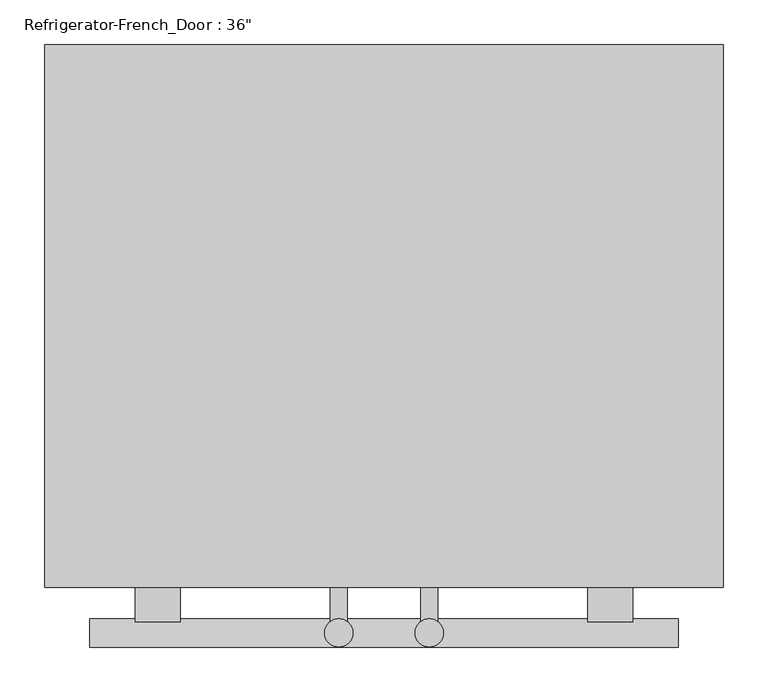
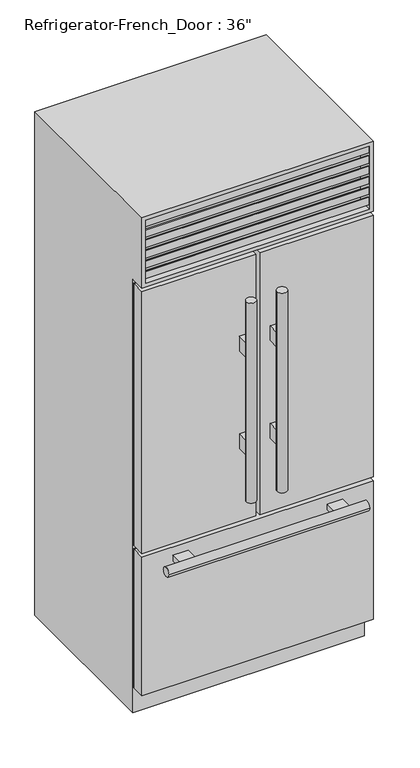
"""IFC4 building model written with IfcOpenShell, lengths in millimetres: proxy geometry."""

from ifc_helpers import new_model, si_unit, frame, origin, place, context, project, spatial, polyline, circle_curve, ellipse_curve, outline, extrude, faceted_brep, source, transform, mapped, element, save
from ifc_brep_helpers import plane_surface, cylinder_surface, advanced_brep


def proxy_12af27c3(model_context):
    return source(origin(), model_context, "Body", "SolidModel", [
        extrude(outline(polyline([(-381.0, -666.75), (-6.35, -666.75), (-6.35, -711.2), (-381.0, -711.2), (-381.0, -666.75)])), frame((0.0, 0.0, 584.2), z_axis=(0.0, 0.0, 1.0), x_axis=(1.0, 0.0, 0.0)), (0.0, 0.0, 1.0), 911.225),
        extrude(outline(polyline([(6.35, -666.75), (381.0, -666.75), (381.0, -711.2), (6.35, -711.2), (6.35, -666.75)])), frame((0.0, 0.0, 584.2), z_axis=(0.0, 0.0, 1.0), x_axis=(1.0, 0.0, 0.0)), (0.0, 0.0, 1.0), 911.225),
        extrude(outline(polyline([(-381.0, -666.75), (381.0, -666.75), (381.0, -711.2), (-381.0, -711.2), (-381.0, -666.75)])), frame((0.0, 0.0, 88.9), z_axis=(0.0, 0.0, 1.0), x_axis=(1.0, 0.0, 0.0)), (0.0, 0.0, 1.0), 482.6),
        faceted_brep([(381.0, -711.2, 1752.6), (-381.0, -711.2, 1752.6), (-381.0, -711.2, 1508.125), (381.0, -711.2, 1508.125), (368.3, -711.2, 1739.9), (368.3, -711.2, 1520.825), (-368.3, -711.2, 1520.825), (-368.3, -711.2, 1739.9), (381.0, -101.6, 1752.6), (-381.0, -101.6, 1752.6), (-381.0, -101.6, 0.0), (-381.0, -660.4, 0.0), (-381.0, -660.4, 1508.125), (381.0, -660.4, 1508.125), (381.0, -660.4, 0.0), (381.0, -101.6, 0.0), (-368.3, -660.4, 1739.9), (368.3, -660.4, 1739.9), (-368.3, -660.4, 1520.825), (368.3, -660.4, 1520.825)], [[[0, 1, 2, 3], [4, 5, 6, 7]], [[1, 0, 8, 9]], [[2, 1, 9, 10, 11, 12]], [[3, 2, 12, 13]], [[8, 0, 3, 13, 14, 15]], [[4, 7, 16, 17]], [[7, 6, 18, 16]], [[6, 5, 19, 18]], [[5, 4, 17, 19]], [[15, 14, 11, 10]], [[9, 8, 15, 10]], [[17, 16, 18, 19]], [[11, 14, 13, 12]]]),
        extrude(outline(polyline([(-660.4, 1520.825), (-708.025, 1533.5860803), (-708.025, 1558.9860803), (-704.85, 1558.9860803), (-704.85, 1536.1368938), (-660.4, 1524.2265522), (-660.4, 1520.825)])), frame((-368.3, 0.0, 0.0), z_axis=(1.0, 0.0, 0.0), x_axis=(0.0, 1.0, 0.0)), (0.0, 0.0, 1.0), 736.6),
        extrude(outline(polyline([(-660.4, 1557.0077839), (-708.025, 1569.7688642), (-708.025, 1595.1688642), (-704.85, 1595.1688642), (-704.85, 1572.3196777), (-660.4, 1560.4093361), (-660.4, 1557.0077839)])), frame((-368.3, 0.0, 0.0), z_axis=(1.0, 0.0, 0.0), x_axis=(0.0, 1.0, 0.0)), (0.0, 0.0, 1.0), 736.6),
        extrude(outline(polyline([(-660.4, 1593.1905679), (-708.025, 1605.9516482), (-708.025, 1631.3516482), (-704.85, 1631.3516482), (-704.85, 1608.5024616), (-660.4, 1596.59212), (-660.4, 1593.1905679)])), frame((-368.3, 0.0, 0.0), z_axis=(1.0, 0.0, 0.0), x_axis=(0.0, 1.0, 0.0)), (0.0, 0.0, 1.0), 736.6),
        extrude(outline(polyline([(-660.4, 1629.3733518), (-708.025, 1642.1344321), (-708.025, 1667.5344321), (-704.85, 1667.5344321), (-704.85, 1644.6852456), (-660.4, 1632.774904), (-660.4, 1629.3733518)])), frame((-368.3, 0.0, 0.0), z_axis=(1.0, 0.0, 0.0), x_axis=(0.0, 1.0, 0.0)), (0.0, 0.0, 1.0), 736.6),
        extrude(outline(polyline([(-660.4, 1665.5561358), (-708.025, 1678.3172161), (-708.025, 1703.7172161), (-704.85, 1703.7172161), (-704.85, 1680.8680295), (-660.4, 1668.9576879), (-660.4, 1665.5561358)])), frame((-368.3, 0.0, 0.0), z_axis=(1.0, 0.0, 0.0), x_axis=(0.0, 1.0, 0.0)), (0.0, 0.0, 1.0), 736.6),
        extrude(outline(polyline([(-660.4, 1701.7389197), (-708.025, 1714.5), (-708.025, 1739.9), (-704.85, 1739.9), (-704.85, 1717.0508135), (-660.4, 1705.1404719), (-660.4, 1701.7389197)])), frame((-368.3, 0.0, 0.0), z_axis=(1.0, 0.0, 0.0), x_axis=(0.0, 1.0, 0.0)), (0.0, 0.0, 1.0), 736.6),
        advanced_brep(
        [(-374.65, -660.4, 565.15), (-374.65, -666.75, 565.15), (-374.65, -666.75, 95.25), (-374.65, -660.4, 95.25), (-377.825, -666.75, 568.325), (-377.825, -660.4, 568.325), (-377.825, -660.4, 92.075), (-377.825, -666.75, 92.075), (374.65, -666.75, 95.25), (374.65, -660.4, 95.25), (377.825, -660.4, 92.075), (377.825, -666.75, 92.075), (374.65, -666.75, 565.15), (374.65, -660.4, 565.15), (377.825, -660.4, 568.325), (377.825, -666.75, 568.325)],
        [
            (0, 1),
            (1, 2),
            (2, 3),
            (3, 0),
            (4, 5, ellipse_curve(frame((-377.825, -663.575, 568.325), z_axis=(-0.7071067811865475, 0.0, -0.7071067811865475), x_axis=(-0.7071067811865474, 0.0, 0.7071067811865476)), 4.4901281, 3.175)),
            (5, 6),
            (6, 7, ellipse_curve(frame((-377.825, -663.575, 92.075), z_axis=(-0.7071067811865475, 0.0, 0.7071067811865475), x_axis=(0.7071067811865474, 0.0, 0.7071067811865476)), 4.4901281, 3.175)),
            (7, 4),
            (2, 8),
            (8, 9),
            (9, 3),
            (6, 10),
            (10, 11, ellipse_curve(frame((377.825, -663.575, 92.075), z_axis=(-0.7071067811865475, 0.0, -0.7071067811865475), x_axis=(-0.7071067811865476, 0.0, 0.7071067811865474)), 4.4901281, 3.175)),
            (11, 7),
            (8, 12),
            (12, 13),
            (13, 9),
            (10, 14),
            (14, 15, ellipse_curve(frame((377.825, -663.575, 568.325), z_axis=(0.7071067811865475, 0.0, -0.7071067811865475), x_axis=(-0.7071067811865474, 0.0, -0.7071067811865476)), 4.4901281, 3.175)),
            (15, 11),
            (12, 1),
            (0, 13),
            (5, 14),
            (4, 15),
        ],
        [
            plane_surface(frame((-374.65, -666.75, 565.15), z_axis=(1.0, 0.0, 0.0), x_axis=(0.0, 0.0, -1.0))),
            cylinder_surface(frame((-377.825, -663.575, 571.5), z_axis=(0.0, 0.0, 1.0), x_axis=(0.0, -1.0, 0.0)), 3.175),
            plane_surface(frame((-374.65, -666.75, 95.25), z_axis=(0.0, 0.0, 1.0), x_axis=(1.0, 0.0, 0.0))),
            cylinder_surface(frame((-381.0, -663.575, 92.075), z_axis=(-1.0, 0.0, 0.0), x_axis=(0.0, -1.0, 0.0)), 3.175),
            plane_surface(frame((374.65, -666.75, 95.25), z_axis=(-1.0, 0.0, 0.0), x_axis=(0.0, 0.0, 1.0))),
            cylinder_surface(frame((377.825, -663.575, 88.9), z_axis=(0.0, 0.0, -1.0), x_axis=(0.0, -1.0, 0.0)), 3.175),
            plane_surface(frame((374.65, -666.75, 565.15), z_axis=(0.0, 0.0, -1.0), x_axis=(-1.0, 0.0, 0.0))),
            plane_surface(frame((374.65, -660.4, 565.15), z_axis=(0.0, 1.0, 0.0), x_axis=(-1.0, 0.0, 0.0))),
            cylinder_surface(frame((381.0, -663.575, 568.325), z_axis=(1.0, 0.0, 0.0), x_axis=(0.0, -1.0, 0.0)), 3.175),
            plane_surface(frame((377.825, -666.75, 568.325), z_axis=(0.0, -1.0, 0.0), x_axis=(-1.0, 0.0, 0.0))),
        ],
        [
            (0, [[1, 2, 3, 4]]),
            (1, [[5, 6, 7, 8]]),
            (2, [[-3, 9, 10, 11]]),
            (3, [[-7, 12, 13, 14]]),
            (4, [[-10, 15, 16, 17]]),
            (5, [[-13, 18, 19, 20]]),
            (6, [[-16, 21, -1, 22]]),
            (7, [[23, -18, -12, -6], [-11, -17, -22, -4]]),
            (8, [[-19, -23, -5, 24]]),
            (9, [[-14, -20, -24, -8], [-21, -15, -9, -2]]),
        ],
    ),
        advanced_brep(
        [(12.7, -660.4, 1489.075), (12.7, -666.75, 1489.075), (12.7, -666.75, 590.55), (12.7, -660.4, 590.55), (9.525, -666.75, 1492.25), (9.525, -660.4, 1492.25), (9.525, -660.4, 587.375), (9.525, -666.75, 587.375), (374.65, -666.75, 590.55), (374.65, -660.4, 590.55), (377.825, -660.4, 587.375), (377.825, -666.75, 587.375), (374.65, -666.75, 1489.075), (374.65, -660.4, 1489.075), (377.825, -660.4, 1492.25), (377.825, -666.75, 1492.25)],
        [
            (0, 1),
            (1, 2),
            (2, 3),
            (3, 0),
            (4, 5, ellipse_curve(frame((9.525, -663.575, 1492.25), z_axis=(-0.7071067811865475, 0.0, -0.7071067811865475), x_axis=(-0.7071067811865474, 0.0, 0.7071067811865476)), 4.4901281, 3.175)),
            (5, 6),
            (6, 7, ellipse_curve(frame((9.525, -663.575, 587.375), z_axis=(-0.7071067811865475, 0.0, 0.7071067811865475), x_axis=(0.7071067811865474, 0.0, 0.7071067811865476)), 4.4901281, 3.175)),
            (7, 4),
            (2, 8),
            (8, 9),
            (9, 3),
            (6, 10),
            (10, 11, ellipse_curve(frame((377.825, -663.575, 587.375), z_axis=(-0.7071067811865475, 0.0, -0.7071067811865475), x_axis=(-0.7071067811865477, 0.0, 0.7071067811865474)), 4.4901281, 3.175)),
            (11, 7),
            (8, 12),
            (12, 13),
            (13, 9),
            (10, 14),
            (14, 15, ellipse_curve(frame((377.825, -663.575, 1492.25), z_axis=(0.7071067811865475, 0.0, -0.7071067811865475), x_axis=(-0.7071067811865474, 0.0, -0.7071067811865477)), 4.4901281, 3.175)),
            (15, 11),
            (12, 1),
            (0, 13),
            (5, 14),
            (4, 15),
        ],
        [
            plane_surface(frame((12.7, -666.75, 1489.075), z_axis=(1.0, 0.0, 0.0), x_axis=(0.0, 0.0, -1.0))),
            cylinder_surface(frame((9.525, -663.575, 1495.425), z_axis=(0.0, 0.0, 1.0), x_axis=(0.0, -1.0, 0.0)), 3.175),
            plane_surface(frame((12.7, -666.75, 590.55), z_axis=(0.0, 0.0, 1.0), x_axis=(1.0, 0.0, 0.0))),
            cylinder_surface(frame((6.35, -663.575, 587.375), z_axis=(-1.0, 0.0, 0.0), x_axis=(0.0, -1.0, 0.0)), 3.175),
            plane_surface(frame((374.65, -666.75, 590.55), z_axis=(-1.0, 0.0, 0.0), x_axis=(0.0, 0.0, 1.0))),
            cylinder_surface(frame((377.825, -663.575, 584.2), z_axis=(0.0, 0.0, -1.0), x_axis=(0.0, -1.0, 0.0)), 3.175),
            plane_surface(frame((374.65, -666.75, 1489.075), z_axis=(0.0, 0.0, -1.0), x_axis=(-1.0, 0.0, 0.0))),
            plane_surface(frame((374.65, -660.4, 1489.075), z_axis=(0.0, 1.0, 0.0), x_axis=(-1.0, 0.0, 0.0))),
            cylinder_surface(frame((381.0, -663.575, 1492.25), z_axis=(1.0, 0.0, 0.0), x_axis=(0.0, -1.0, 0.0)), 3.175),
            plane_surface(frame((377.825, -666.75, 1492.25), z_axis=(0.0, -1.0, 0.0), x_axis=(-1.0, 0.0, 0.0))),
        ],
        [
            (0, [[1, 2, 3, 4]]),
            (1, [[5, 6, 7, 8]]),
            (2, [[-3, 9, 10, 11]]),
            (3, [[-7, 12, 13, 14]]),
            (4, [[-10, 15, 16, 17]]),
            (5, [[-13, 18, 19, 20]]),
            (6, [[-16, 21, -1, 22]]),
            (7, [[23, -18, -12, -6], [-11, -17, -22, -4]]),
            (8, [[-19, -23, -5, 24]]),
            (9, [[-14, -20, -24, -8], [-21, -15, -9, -2]]),
        ],
    ),
        advanced_brep(
        [(-374.65, -660.4, 1489.075), (-374.65, -666.75, 1489.075), (-374.65, -666.75, 590.55), (-374.65, -660.4, 590.55), (-377.825, -666.75, 1492.25), (-377.825, -660.4, 1492.25), (-377.825, -660.4, 587.375), (-377.825, -666.75, 587.375), (-12.7, -666.75, 590.55), (-12.7, -660.4, 590.55), (-9.525, -660.4, 587.375), (-9.525, -666.75, 587.375), (-12.7, -666.75, 1489.075), (-12.7, -660.4, 1489.075), (-9.525, -660.4, 1492.25), (-9.525, -666.75, 1492.25)],
        [
            (0, 1),
            (1, 2),
            (2, 3),
            (3, 0),
            (4, 5, ellipse_curve(frame((-377.825, -663.575, 1492.25), z_axis=(-0.7071067811865476, 0.0, -0.7071067811865475), x_axis=(-0.7071067811865474, 0.0, 0.7071067811865476)), 4.4901281, 3.175)),
            (5, 6),
            (6, 7, ellipse_curve(frame((-377.825, -663.575, 587.375), z_axis=(-0.7071067811865475, 0.0, 0.7071067811865475), x_axis=(0.7071067811865474, 0.0, 0.7071067811865476)), 4.4901281, 3.175)),
            (7, 4),
            (2, 8),
            (8, 9),
            (9, 3),
            (6, 10),
            (10, 11, ellipse_curve(frame((-9.525, -663.575, 587.375), z_axis=(-0.7071067811865475, 0.0, -0.7071067811865475), x_axis=(-0.7071067811865476, 0.0, 0.7071067811865474)), 4.4901281, 3.175)),
            (11, 7),
            (8, 12),
            (12, 13),
            (13, 9),
            (10, 14),
            (14, 15, ellipse_curve(frame((-9.525, -663.575, 1492.25), z_axis=(0.7071067811865475, 0.0, -0.7071067811865475), x_axis=(-0.7071067811865474, 0.0, -0.7071067811865476)), 4.4901281, 3.175)),
            (15, 11),
            (12, 1),
            (0, 13),
            (5, 14),
            (4, 15),
        ],
        [
            plane_surface(frame((-374.65, -666.75, 1489.075), z_axis=(1.0, 0.0, 0.0), x_axis=(0.0, 0.0, -1.0))),
            cylinder_surface(frame((-377.825, -663.575, 1495.425), z_axis=(0.0, 0.0, 1.0), x_axis=(0.0, -1.0, 0.0)), 3.175),
            plane_surface(frame((-374.65, -666.75, 590.55), z_axis=(0.0, 0.0, 1.0), x_axis=(1.0, 0.0, 0.0))),
            cylinder_surface(frame((-381.0, -663.575, 587.375), z_axis=(-1.0, 0.0, 0.0), x_axis=(0.0, -1.0, 0.0)), 3.175),
            plane_surface(frame((-12.7, -666.75, 590.55), z_axis=(-1.0, 0.0, 0.0), x_axis=(0.0, 0.0, 1.0))),
            cylinder_surface(frame((-9.525, -663.575, 584.2), z_axis=(0.0, 0.0, -1.0), x_axis=(0.0, -1.0, 0.0)), 3.175),
            plane_surface(frame((-12.7, -666.75, 1489.075), z_axis=(0.0, 0.0, -1.0), x_axis=(-1.0, 0.0, 0.0))),
            plane_surface(frame((-12.7, -660.4, 1489.075), z_axis=(0.0, 1.0, 0.0), x_axis=(-1.0, 0.0, 0.0))),
            cylinder_surface(frame((-6.35, -663.575, 1492.25), z_axis=(1.0, 0.0, 0.0), x_axis=(0.0, -1.0, 0.0)), 3.175),
            plane_surface(frame((-9.525, -666.75, 1492.25), z_axis=(0.0, -1.0, 0.0), x_axis=(-1.0, 0.0, 0.0))),
        ],
        [
            (0, [[1, 2, 3, 4]]),
            (1, [[5, 6, 7, 8]]),
            (2, [[-3, 9, 10, 11]]),
            (3, [[-7, 12, 13, 14]]),
            (4, [[-10, 15, 16, 17]]),
            (5, [[-13, 18, 19, 20]]),
            (6, [[-16, 21, -1, 22]]),
            (7, [[23, -18, -12, -6], [-11, -17, -22, -4]]),
            (8, [[-19, -23, -5, 24]]),
            (9, [[-14, -20, -24, -8], [-21, -15, -9, -2]]),
        ],
    ),
        advanced_brep(
        [(-228.6, -711.2, 542.925), (-228.6, -711.2, 523.875), (-279.4, -711.2, 523.875), (-279.4, -711.2, 542.925), (228.6, -711.2, 542.925), (279.4, -711.2, 542.925), (279.4, -711.2, 523.875), (228.6, -711.2, 523.875), (-228.6, -749.6741958, 542.925), (-228.6, -746.4991958, 533.4), (-228.6, -749.6741958, 523.875), (-279.4, -749.6741958, 523.875), (-279.4, -746.4991958, 533.4), (-279.4, -749.6741958, 542.925), (228.6, -749.6741958, 542.925), (279.4, -749.6741958, 542.925), (279.4, -746.4991958, 533.4), (279.4, -749.6741958, 523.875), (228.6, -749.6741958, 523.875), (228.6, -746.4991958, 533.4), (330.2, -778.2491958, 533.4), (330.2, -746.4991958, 533.4), (-330.2, -778.2491958, 533.4), (-330.2, -746.4991958, 533.4)],
        [
            (0, 1),
            (1, 2),
            (2, 3),
            (3, 0),
            (4, 5),
            (5, 6),
            (6, 7),
            (7, 4),
            (0, 8),
            (8, 9, circle_curve(frame((-228.6, -762.3741958, 533.4), z_axis=(-1.0, 0.0, 0.0), x_axis=(0.0, 1.0, 0.0)), 15.875)),
            (9, 10, circle_curve(frame((-228.6, -762.3741958, 533.4), z_axis=(-1.0, 0.0, 0.0), x_axis=(0.0, 1.0, 0.0)), 15.875)),
            (10, 1),
            (10, 11),
            (11, 2),
            (11, 12, circle_curve(frame((-279.4, -762.3741958, 533.4), z_axis=(1.0, 0.0, 0.0), x_axis=(0.0, 1.0, 0.0)), 15.875)),
            (12, 13, circle_curve(frame((-279.4, -762.3741958, 533.4), z_axis=(1.0, 0.0, 0.0), x_axis=(0.0, 1.0, 0.0)), 15.875)),
            (13, 3),
            (13, 8),
            (4, 14),
            (14, 15),
            (15, 5),
            (15, 16, circle_curve(frame((279.4, -762.3741958, 533.4), z_axis=(-1.0, 0.0, 0.0), x_axis=(0.0, 1.0, 0.0)), 15.875)),
            (16, 17, circle_curve(frame((279.4, -762.3741958, 533.4), z_axis=(-1.0, 0.0, 0.0), x_axis=(0.0, 1.0, 0.0)), 15.875)),
            (17, 6),
            (17, 18),
            (18, 7),
            (18, 19, circle_curve(frame((228.6, -762.3741958, 533.4), z_axis=(1.0, 0.0, 0.0), x_axis=(0.0, 1.0, 0.0)), 15.875)),
            (19, 14, circle_curve(frame((228.6, -762.3741958, 533.4), z_axis=(1.0, 0.0, 0.0), x_axis=(0.0, 1.0, 0.0)), 15.875)),
            (20, 21, circle_curve(frame((330.2, -762.3741958, 533.4), z_axis=(1.0, 0.0, 0.0), x_axis=(0.0, 1.0, 0.0)), 15.875)),
            (21, 20, circle_curve(frame((330.2, -762.3741958, 533.4), z_axis=(1.0, 0.0, 0.0), x_axis=(0.0, 1.0, 0.0)), 15.875)),
            (22, 23, circle_curve(frame((-330.2, -762.3741958, 533.4), z_axis=(-1.0, 0.0, 0.0), x_axis=(0.0, 1.0, 0.0)), 15.875)),
            (23, 22, circle_curve(frame((-330.2, -762.3741958, 533.4), z_axis=(-1.0, 0.0, 0.0), x_axis=(0.0, 1.0, 0.0)), 15.875)),
            (20, 22),
            (23, 12),
            (9, 19),
            (16, 21),
        ],
        [
            plane_surface(frame((-228.6, -711.2, 542.925), z_axis=(0.0, 1.0, 0.0), x_axis=(0.0, 0.0, -1.0))),
            plane_surface(frame((-228.6, -711.2, 542.925), z_axis=(1.0, 0.0, 0.0), x_axis=(0.0, -1.0, 0.0))),
            plane_surface(frame((-228.6, -711.2, 523.875), z_axis=(0.0, 0.0, -1.0), x_axis=(0.0, -1.0, 0.0))),
            plane_surface(frame((-279.4, -711.2, 523.875), z_axis=(-1.0, 0.0, 0.0), x_axis=(0.0, -1.0, 0.0))),
            plane_surface(frame((-279.4, -711.2, 542.925), z_axis=(0.0, 0.0, 1.0), x_axis=(0.0, -1.0, 0.0))),
            plane_surface(frame((228.6, -711.2, 542.925), z_axis=(0.0, 0.0, 1.0), x_axis=(0.0, -1.0, 0.0))),
            plane_surface(frame((279.4, -711.2, 542.925), z_axis=(1.0, 0.0, 0.0), x_axis=(0.0, -1.0, 0.0))),
            plane_surface(frame((279.4, -711.2, 523.875), z_axis=(0.0, 0.0, -1.0), x_axis=(0.0, -1.0, 0.0))),
            plane_surface(frame((228.6, -711.2, 523.875), z_axis=(-1.0, 0.0, 0.0), x_axis=(0.0, -1.0, 0.0))),
            plane_surface(frame((330.2, -746.4991958, 533.4), z_axis=(1.0, 0.0, 0.0), x_axis=(0.0, 0.0, 1.0))),
            plane_surface(frame((-330.2, -746.4991958, 533.4), z_axis=(-1.0, 0.0, 0.0), x_axis=(0.0, 0.0, -1.0))),
            cylinder_surface(frame((-330.2, -762.3741958, 533.4), z_axis=(1.0, 0.0, 0.0), x_axis=(0.0, 1.0, 0.0)), 15.875),
        ],
        [
            (0, [[1, 2, 3, 4]]),
            (0, [[5, 6, 7, 8]]),
            (1, [[-1, 9, 10, 11, 12]]),
            (2, [[-2, -12, 13, 14]]),
            (3, [[-3, -14, 15, 16, 17]]),
            (4, [[-4, -17, 18, -9]]),
            (5, [[-5, 19, 20, 21]]),
            (6, [[-6, -21, 22, 23, 24]]),
            (7, [[-7, -24, 25, 26]]),
            (8, [[-8, -26, 27, 28, -19]]),
            (9, [[29, 30]]),
            (10, [[31, 32]]),
            (11, [[-29, 33, -32, 34, -15, -13, -11, 35, -27, -25, -23, 36]]),
            (11, [[-30, -36, -22, -20, -28, -35, -10, -18, -16, -34, -31, -33]]),
        ],
    ),
        advanced_brep(
        [(34.925, -762.3741958, 1381.125), (66.675, -762.3741958, 1381.125), (34.925, -762.3741958, 685.8), (66.675, -762.3741958, 685.8), (60.325, -749.6741958, 1177.925), (60.325, -749.6741958, 1228.725), (41.275, -749.6741958, 1228.725), (41.275, -749.6741958, 1177.925), (60.325, -749.6741958, 838.2), (60.325, -749.6741958, 889.0), (41.275, -749.6741958, 889.0), (41.275, -749.6741958, 838.2), (60.325, -711.2, 1228.725), (60.325, -711.2, 1177.925), (41.275, -711.2, 1177.925), (41.275, -711.2, 1228.725), (60.325, -711.2, 889.0), (60.325, -711.2, 838.2), (41.275, -711.2, 838.2), (41.275, -711.2, 889.0)],
        [
            (0, 1, circle_curve(frame((50.8, -762.3741958, 1381.125), z_axis=(0.0, 0.0, 1.0), x_axis=(1.0, 0.0, 0.0)), 15.875)),
            (1, 0, circle_curve(frame((50.8, -762.3741958, 1381.125), z_axis=(0.0, 0.0, 1.0), x_axis=(1.0, 0.0, 0.0)), 15.875)),
            (2, 3, circle_curve(frame((50.8, -762.3741958, 685.8), z_axis=(0.0, 0.0, -1.0), x_axis=(1.0, 0.0, 0.0)), 15.875)),
            (3, 2, circle_curve(frame((50.8, -762.3741958, 685.8), z_axis=(0.0, 0.0, -1.0), x_axis=(1.0, 0.0, 0.0)), 15.875)),
            (0, 2),
            (3, 1),
            (4, 5),
            (5, 6, circle_curve(frame((50.8, -762.3741958, 1228.725), z_axis=(0.0, 0.0, 1.0), x_axis=(1.0, 0.0, 0.0)), 15.875)),
            (6, 7),
            (7, 4, circle_curve(frame((50.8, -762.3741958, 1177.925), z_axis=(0.0, 0.0, -1.0), x_axis=(1.0, 0.0, 0.0)), 15.875)),
            (8, 9),
            (9, 10, circle_curve(frame((50.8, -762.3741958, 889.0), z_axis=(0.0, 0.0, 1.0), x_axis=(1.0, 0.0, 0.0)), 15.875)),
            (10, 11),
            (11, 8, circle_curve(frame((50.8, -762.3741958, 838.2), z_axis=(0.0, 0.0, -1.0), x_axis=(1.0, 0.0, 0.0)), 15.875)),
            (12, 13),
            (13, 14),
            (14, 15),
            (15, 12),
            (16, 17),
            (17, 18),
            (18, 19),
            (19, 16),
            (12, 5),
            (4, 13),
            (7, 14),
            (6, 15),
            (16, 9),
            (8, 17),
            (11, 18),
            (10, 19),
        ],
        [
            plane_surface(frame((66.675, -762.3741958, 1381.125), z_axis=(0.0, 0.0, 1.0), x_axis=(0.0, 1.0, 0.0))),
            plane_surface(frame((66.675, -762.3741958, 685.8), z_axis=(0.0, 0.0, -1.0), x_axis=(0.0, -1.0, 0.0))),
            cylinder_surface(frame((50.8, -762.3741958, 685.8), z_axis=(0.0, 0.0, 1.0), x_axis=(1.0, 0.0, 0.0)), 15.875),
            plane_surface(frame((60.325, -711.2, 1228.725), z_axis=(0.0, 1.0, 0.0), x_axis=(0.0, 0.0, -1.0))),
            plane_surface(frame((60.325, -711.2, 1228.725), z_axis=(1.0, 0.0, 0.0), x_axis=(0.0, -1.0, 0.0))),
            plane_surface(frame((60.325, -711.2, 1177.925), z_axis=(0.0, 0.0, -1.0), x_axis=(0.0, -1.0, 0.0))),
            plane_surface(frame((41.275, -711.2, 1177.925), z_axis=(-1.0, 0.0, 0.0), x_axis=(0.0, -1.0, 0.0))),
            plane_surface(frame((41.275, -711.2, 1228.725), z_axis=(0.0, 0.0, 1.0), x_axis=(0.0, -1.0, 0.0))),
            plane_surface(frame((60.325, -711.2, 889.0), z_axis=(1.0, 0.0, 0.0), x_axis=(0.0, -1.0, 0.0))),
            plane_surface(frame((60.325, -711.2, 838.2), z_axis=(0.0, 0.0, -1.0), x_axis=(0.0, -1.0, 0.0))),
            plane_surface(frame((41.275, -711.2, 838.2), z_axis=(-1.0, 0.0, 0.0), x_axis=(0.0, -1.0, 0.0))),
            plane_surface(frame((41.275, -711.2, 889.0), z_axis=(0.0, 0.0, 1.0), x_axis=(0.0, -1.0, 0.0))),
        ],
        [
            (0, [[1, 2]]),
            (1, [[3, 4]]),
            (2, [[-1, 5, -4, 6]]),
            (2, [[-2, -6, -3, -5], [7, 8, 9, 10], [11, 12, 13, 14]]),
            (3, [[15, 16, 17, 18]]),
            (3, [[19, 20, 21, 22]]),
            (4, [[-15, 23, -7, 24]]),
            (5, [[-16, -24, -10, 25]]),
            (6, [[-17, -25, -9, 26]]),
            (7, [[-18, -26, -8, -23]]),
            (8, [[-19, 27, -11, 28]]),
            (9, [[-20, -28, -14, 29]]),
            (10, [[-21, -29, -13, 30]]),
            (11, [[-22, -30, -12, -27]]),
        ],
    ),
        advanced_brep(
        [(-41.275, -711.2, 1228.725), (-41.275, -711.2, 1177.925), (-60.325, -711.2, 1177.925), (-60.325, -711.2, 1228.725), (-41.275, -711.2, 889.0), (-41.275, -711.2, 838.2), (-60.325, -711.2, 838.2), (-60.325, -711.2, 889.0), (-41.275, -749.6741958, 1228.725), (-41.275, -749.6741958, 1177.925), (-60.325, -749.6741958, 1177.925), (-60.325, -749.6741958, 1228.725), (-41.275, -749.6741958, 889.0), (-41.275, -749.6741958, 838.2), (-60.325, -749.6741958, 838.2), (-60.325, -749.6741958, 889.0), (-66.675, -762.3741958, 1381.125), (-34.925, -762.3741958, 1381.125), (-66.675, -762.3741958, 685.8), (-34.925, -762.3741958, 685.8)],
        [
            (0, 1),
            (1, 2),
            (2, 3),
            (3, 0),
            (4, 5),
            (5, 6),
            (6, 7),
            (7, 4),
            (0, 8),
            (8, 9),
            (9, 1),
            (9, 10, circle_curve(frame((-50.8, -762.3741958, 1177.925), z_axis=(0.0, 0.0, 1.0), x_axis=(1.0, 0.0, 0.0)), 15.875)),
            (10, 2),
            (10, 11),
            (11, 3),
            (11, 8, circle_curve(frame((-50.8, -762.3741958, 1228.725), z_axis=(0.0, 0.0, -1.0), x_axis=(1.0, 0.0, 0.0)), 15.875)),
            (4, 12),
            (12, 13),
            (13, 5),
            (13, 14, circle_curve(frame((-50.8, -762.3741958, 838.2), z_axis=(0.0, 0.0, 1.0), x_axis=(1.0, 0.0, 0.0)), 15.875)),
            (14, 6),
            (14, 15),
            (15, 7),
            (15, 12, circle_curve(frame((-50.8, -762.3741958, 889.0), z_axis=(0.0, 0.0, -1.0), x_axis=(1.0, 0.0, 0.0)), 15.875)),
            (16, 17, circle_curve(frame((-50.8, -762.3741958, 1381.125), z_axis=(0.0, 0.0, 1.0), x_axis=(1.0, 0.0, 0.0)), 15.875)),
            (17, 16, circle_curve(frame((-50.8, -762.3741958, 1381.125), z_axis=(0.0, 0.0, 1.0), x_axis=(1.0, 0.0, 0.0)), 15.875)),
            (18, 19, circle_curve(frame((-50.8, -762.3741958, 685.8), z_axis=(0.0, 0.0, -1.0), x_axis=(1.0, 0.0, 0.0)), 15.875)),
            (19, 18, circle_curve(frame((-50.8, -762.3741958, 685.8), z_axis=(0.0, 0.0, -1.0), x_axis=(1.0, 0.0, 0.0)), 15.875)),
            (16, 18),
            (19, 17),
        ],
        [
            plane_surface(frame((-41.275, -711.2, 1228.725), z_axis=(0.0, 1.0, 0.0), x_axis=(0.0, 0.0, -1.0))),
            plane_surface(frame((-41.275, -711.2, 1228.725), z_axis=(1.0, 0.0, 0.0), x_axis=(0.0, -1.0, 0.0))),
            plane_surface(frame((-41.275, -711.2, 1177.925), z_axis=(0.0, 0.0, -1.0), x_axis=(0.0, -1.0, 0.0))),
            plane_surface(frame((-60.325, -711.2, 1177.925), z_axis=(-1.0, 0.0, 0.0), x_axis=(0.0, -1.0, 0.0))),
            plane_surface(frame((-60.325, -711.2, 1228.725), z_axis=(0.0, 0.0, 1.0), x_axis=(0.0, -1.0, 0.0))),
            plane_surface(frame((-41.275, -711.2, 889.0), z_axis=(1.0, 0.0, 0.0), x_axis=(0.0, -1.0, 0.0))),
            plane_surface(frame((-41.275, -711.2, 838.2), z_axis=(0.0, 0.0, -1.0), x_axis=(0.0, -1.0, 0.0))),
            plane_surface(frame((-60.325, -711.2, 838.2), z_axis=(-1.0, 0.0, 0.0), x_axis=(0.0, -1.0, 0.0))),
            plane_surface(frame((-60.325, -711.2, 889.0), z_axis=(0.0, 0.0, 1.0), x_axis=(0.0, -1.0, 0.0))),
            plane_surface(frame((-34.925, -762.3741958, 1381.125), z_axis=(0.0, 0.0, 1.0), x_axis=(0.0, 1.0, 0.0))),
            plane_surface(frame((-34.925, -762.3741958, 685.8), z_axis=(0.0, 0.0, -1.0), x_axis=(0.0, -1.0, 0.0))),
            cylinder_surface(frame((-50.8, -762.3741958, 685.8), z_axis=(0.0, 0.0, 1.0), x_axis=(1.0, 0.0, 0.0)), 15.875),
        ],
        [
            (0, [[1, 2, 3, 4]]),
            (0, [[5, 6, 7, 8]]),
            (1, [[-1, 9, 10, 11]]),
            (2, [[-2, -11, 12, 13]]),
            (3, [[-3, -13, 14, 15]]),
            (4, [[-4, -15, 16, -9]]),
            (5, [[-5, 17, 18, 19]]),
            (6, [[-6, -19, 20, 21]]),
            (7, [[-7, -21, 22, 23]]),
            (8, [[-8, -23, 24, -17]]),
            (9, [[25, 26]]),
            (10, [[27, 28]]),
            (11, [[-25, 29, -28, 30]]),
            (11, [[-26, -30, -27, -29], [-10, -16, -14, -12], [-18, -24, -22, -20]]),
        ],
    ),
    ])


if __name__ == "__main__":
    model = new_model("IFC4")
    model_context = context("Model", 3, world=origin())
    ifc_project = project(units=[si_unit("LENGTHUNIT", "METRE", prefix="MILLI")], contexts=[model_context])
    site = spatial("IfcSite", under=ifc_project)
    building = spatial("IfcBuilding", under=site)
    placement = place(None, origin())
    proxy_shape = proxy_12af27c3(model_context)
    element("IfcBuildingElementProxy", 1, Name="Refrigerator-French_Door : 36\"", ObjectType="Refrigerator-French_Door : 36\"", at=placement, inside=building, context=model_context, shape_type="MappedRepresentation", body=[
        mapped(proxy_shape, transform((0.0, 0.0, 0.0), x_axis=(1.0, 0.0, 0.0), y_axis=(0.0, 1.0, 0.0), z_axis=(0.0, 0.0, 1.0))),
    ])
    save(model, "model.ifc")

# Revit data of these elements
# Type "Refrigerator-French_Door : 36\""
#   Label = "Refrigerator"
#   Description = "French Door Refrigerator"
#   Assembly Code = "E1090320"
#   Door Width = 1' - 2 3/4"
#   Width = 2' - 6"
#   Wall Offset = 0' - 4"
#   Voltage = 120 V
#   Power Consumption = 1000 VA
#   Height = 5' - 9"
#   Depth = 2' - 0"
#   Amperage = 8.33333 A
#   Show Label = yes
#   Gasket = Appliance - Gasket
#   Appliance Finish = Appliance - Stainless Steel
#   Default Elevation = 0
# Element 1 (IfcBuildingElementProxy, "Refrigerator-French_Door : 36\"")
#   Materials on its faces: "Appliance - Stainless Steel", "Appliance - Gasket"
# Materials
#   "Appliance - Gasket": class "Miscellaneous", colour RGB 234 234 234, transparency 0, Cost = 0
#   "Appliance - Stainless Steel": class "Metal", colour RGB 189 187 185, transparency 0, Description = "Stainless Steel 18/8", Cost = 0
